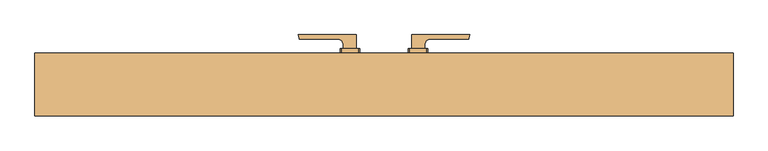
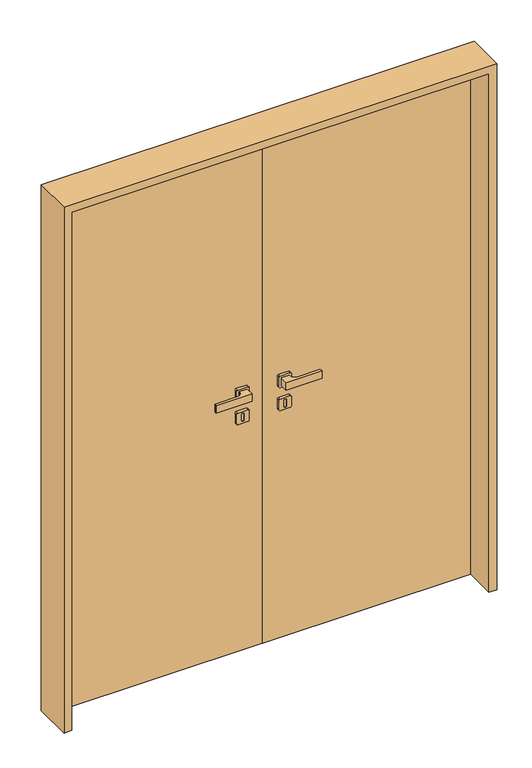
"""IFC4 building model written with IfcOpenShell, lengths in millimetres: door geometry, porta multiplas_growarq : porta giro duplo 80 cm_growarq."""

from ifc_helpers import new_model, si_unit, point, frame, frame_2d, origin, origin_with_axes, place, context, project, spatial, polyline, circle_curve, trimmed, segment, composite_curve, outline, extrude, source, transform, mapped, element, save
from ifc_brep_helpers import plane_surface, cylinder_surface, revolved_surface, advanced_brep


def door_8bf3503e(model_context):
    return source(origin(), model_context, "Body", "SolidModel", [
        advanced_brep(
        [(-61.4752094, 86.0, 975.2140175), (-57.4752094, 86.0, 971.2140175), (-57.4752094, 86.0, 932.3348635), (-61.4752094, 86.0, 928.3348635), (-100.524804, 86.0, 928.3348635), (-104.524804, 86.0, 932.3348635), (-104.524804, 86.0, 971.2071442), (-100.5179308, 86.0, 975.2140175), (-75.9963765, 86.0, 963.1453546), (-86.0064486, 86.0, 963.1453546), (-86.0064486, 86.0, 940.4035264), (-75.9963765, 86.0, 940.4035264), (-61.4752094, 75.0, 975.2140175), (-100.5179308, 75.0, 975.2140175), (-104.524804, 75.0, 971.2071442), (-104.524804, 75.0, 932.3348635), (-100.524804, 75.0, 928.3348635), (-61.4752094, 75.0, 928.3348635), (-57.4752094, 75.0, 932.3348635), (-57.4752094, 75.0, 971.2140175), (-75.9963765, 84.0, 940.4035264), (-86.0064486, 84.0, 940.4035264), (-86.0064486, 84.0, 963.1453546), (-75.9963765, 84.0, 963.1453546)],
        [
            (0, 1, circle_curve(frame((-61.4752094, 86.0, 971.2140175), z_axis=(0.0, 1.0, 0.0), x_axis=(1.0, 0.0, 0.0)), 4.0)),
            (1, 2),
            (2, 3, circle_curve(frame((-61.4752094, 86.0, 932.3348635), z_axis=(0.0, 1.0, 0.0), x_axis=(1.0, 0.0, 0.0)), 4.0)),
            (3, 4),
            (4, 5, circle_curve(frame((-100.524804, 86.0, 932.3348635), z_axis=(0.0, 1.0, 0.0), x_axis=(1.0, 0.0, 0.0)), 4.0)),
            (5, 6),
            (6, 7, circle_curve(frame((-100.5179308, 86.0, 971.2071442), z_axis=(0.0, 1.0, 0.0), x_axis=(1.0, 0.0, 0.0)), 4.0068732)),
            (7, 0),
            (8, 9, circle_curve(frame((-81.0014126, 86.0, 963.1453546), z_axis=(0.0, -1.0, 0.0), x_axis=(1.0, 0.0, 0.0)), 5.0050361)),
            (9, 10),
            (10, 11, circle_curve(frame((-81.0014126, 86.0, 940.4035264), z_axis=(0.0, -1.0, 0.0), x_axis=(1.0, 0.0, 0.0)), 5.0050361)),
            (11, 8),
            (12, 13),
            (13, 14, circle_curve(frame((-100.5179308, 75.0, 971.2071442), z_axis=(0.0, -1.0, 0.0), x_axis=(1.0, 0.0, 0.0)), 4.0068732)),
            (14, 15),
            (15, 16, circle_curve(frame((-100.524804, 75.0, 932.3348635), z_axis=(0.0, -1.0, 0.0), x_axis=(1.0, 0.0, 0.0)), 4.0)),
            (16, 17),
            (17, 18, circle_curve(frame((-61.4752094, 75.0, 932.3348635), z_axis=(0.0, -1.0, 0.0), x_axis=(1.0, 0.0, 0.0)), 4.0)),
            (18, 19),
            (19, 12, circle_curve(frame((-61.4752094, 75.0, 971.2140175), z_axis=(0.0, -1.0, 0.0), x_axis=(1.0, 0.0, 0.0)), 4.0)),
            (7, 13),
            (12, 0),
            (6, 14),
            (5, 15),
            (4, 16),
            (3, 17),
            (2, 18),
            (1, 19),
            (20, 21, circle_curve(frame((-81.0014126, 84.0, 940.4035264), z_axis=(0.0, 1.0, 0.0), x_axis=(1.0, 0.0, 0.0)), 5.0050361)),
            (21, 22),
            (22, 23, circle_curve(frame((-81.0014126, 84.0, 963.1453546), z_axis=(0.0, 1.0, 0.0), x_axis=(1.0, 0.0, 0.0)), 5.0050361)),
            (23, 20),
            (23, 8),
            (11, 20),
            (21, 10),
            (9, 22),
        ],
        [
            plane_surface(frame((-100.5218961, 86.0, 975.2140175), z_axis=(0.0, 1.0, 0.0), x_axis=(-1.0, 0.0, 0.0))),
            plane_surface(frame((-100.5218961, 75.0, 975.2140175), z_axis=(0.0, -1.0, 0.0), x_axis=(1.0, 0.0, 0.0))),
            plane_surface(frame((-61.4752094, 86.0, 975.2140175), z_axis=(0.0, 0.0, 1.0), x_axis=(0.0, -1.0, 0.0))),
            cylinder_surface(frame((-100.5179308, 75.0, 971.2071442), z_axis=(0.0, 1.0, 0.0), x_axis=(1.0, 0.0, 0.0)), 4.0068732),
            plane_surface(frame((-104.524804, 86.0, 971.2071442), z_axis=(-1.0, 0.0, 0.0), x_axis=(0.0, -1.0, 0.0))),
            cylinder_surface(frame((-100.524804, 75.0, 932.3348635), z_axis=(0.0, 1.0, 0.0), x_axis=(1.0, 0.0, 0.0)), 4.0),
            plane_surface(frame((-100.524804, 86.0, 928.3348635), z_axis=(0.0, 0.0, -1.0), x_axis=(0.0, -1.0, 0.0))),
            cylinder_surface(frame((-61.4752094, 75.0, 932.3348635), z_axis=(0.0, 1.0, 0.0), x_axis=(1.0, 0.0, 0.0)), 4.0),
            plane_surface(frame((-57.4752094, 86.0, 932.3348635), z_axis=(1.0, 0.0, 0.0), x_axis=(0.0, -1.0, 0.0))),
            cylinder_surface(frame((-61.4752094, 75.0, 971.2140175), z_axis=(0.0, 1.0, 0.0), x_axis=(1.0, 0.0, 0.0)), 4.0),
            plane_surface(frame((-75.9963765, 84.0, 952.9958878), z_axis=(0.0, 1.0, 0.0), x_axis=(0.0, 0.0, -1.0))),
            plane_surface(frame((-75.9963765, 86.0, 940.4035264), z_axis=(-1.0, 0.0, 0.0), x_axis=(0.0, -1.0, 0.0))),
            plane_surface(frame((-86.0064486, 86.0, 963.1453546), z_axis=(1.0, 0.0, 0.0), x_axis=(0.0, -1.0, 0.0))),
            revolved_surface(polyline([(-75.9963765, 86.0, 940.4035264), (-75.9963765, 84.0, 940.4035264)]), (-81.0014126, 84.0, 940.4035264), (0.0, 1.0, 0.0)),
            revolved_surface(polyline([(-75.9963765, 86.0, 963.1453546), (-75.9963765, 84.0, 963.1453546)]), (-81.0014126, 84.0, 963.1453546), (0.0, 1.0, 0.0)),
        ],
        [
            (0, [[1, 2, 3, 4, 5, 6, 7, 8], [9, 10, 11, 12]]),
            (1, [[13, 14, 15, 16, 17, 18, 19, 20]]),
            (2, [[21, -13, 22, -8]]),
            (3, [[23, -14, -21, -7]]),
            (4, [[24, -15, -23, -6]]),
            (5, [[25, -16, -24, -5]]),
            (6, [[26, -17, -25, -4]]),
            (7, [[27, -18, -26, -3]]),
            (8, [[28, -19, -27, -2]]),
            (9, [[-22, -20, -28, -1]]),
            (10, [[29, 30, 31, 32]]),
            (11, [[33, -12, 34, -32]]),
            (12, [[35, -10, 36, -30]]),
            (13, [[-34, -11, -35, -29]]),
            (14, [[-36, -9, -33, -31]]),
        ],
    ),
        advanced_brep(
        [(-61.4752094, 86.0, 1068.227973), (-57.4752094, 86.0, 1064.227973), (-57.4752094, 86.0, 1025.3488191), (-61.4752094, 86.0, 1021.3488191), (-100.524804, 86.0, 1021.3488191), (-104.524804, 86.0, 1025.3488191), (-104.524804, 86.0, 1064.2210998), (-100.5179308, 86.0, 1068.227973), (-61.4752094, 75.0, 1068.227973), (-100.5179308, 75.0, 1068.227973), (-104.524804, 75.0, 1064.2210998), (-104.524804, 75.0, 1025.3488191), (-100.524804, 75.0, 1021.3488191), (-61.4752094, 75.0, 1021.3488191), (-57.4752094, 75.0, 1025.3488191), (-57.4752094, 75.0, 1064.227973)],
        [
            (0, 1, circle_curve(frame((-61.4752094, 86.0, 1064.227973), z_axis=(0.0, 1.0, 0.0), x_axis=(1.0, 0.0, 0.0)), 4.0)),
            (1, 2),
            (2, 3, circle_curve(frame((-61.4752094, 86.0, 1025.3488191), z_axis=(0.0, 1.0, 0.0), x_axis=(1.0, 0.0, 0.0)), 4.0)),
            (3, 4),
            (4, 5, circle_curve(frame((-100.524804, 86.0, 1025.3488191), z_axis=(0.0, 1.0, 0.0), x_axis=(1.0, 0.0, 0.0)), 4.0)),
            (5, 6),
            (6, 7, circle_curve(frame((-100.5179308, 86.0, 1064.2210998), z_axis=(0.0, 1.0, 0.0), x_axis=(1.0, 0.0, 0.0)), 4.0068732)),
            (7, 0),
            (8, 9),
            (9, 10, circle_curve(frame((-100.5179308, 75.0, 1064.2210998), z_axis=(0.0, -1.0, 0.0), x_axis=(1.0, 0.0, 0.0)), 4.0068732)),
            (10, 11),
            (11, 12, circle_curve(frame((-100.524804, 75.0, 1025.3488191), z_axis=(0.0, -1.0, 0.0), x_axis=(1.0, 0.0, 0.0)), 4.0)),
            (12, 13),
            (13, 14, circle_curve(frame((-61.4752094, 75.0, 1025.3488191), z_axis=(0.0, -1.0, 0.0), x_axis=(1.0, 0.0, 0.0)), 4.0)),
            (14, 15),
            (15, 8, circle_curve(frame((-61.4752094, 75.0, 1064.227973), z_axis=(0.0, -1.0, 0.0), x_axis=(1.0, 0.0, 0.0)), 4.0)),
            (7, 9),
            (8, 0),
            (6, 10),
            (5, 11),
            (4, 12),
            (3, 13),
            (2, 14),
            (1, 15),
        ],
        [
            plane_surface(frame((-100.5218961, 86.0, 975.2140175), z_axis=(0.0, 1.0, 0.0), x_axis=(-1.0, 0.0, 0.0))),
            plane_surface(frame((-100.5218961, 75.0, 975.2140175), z_axis=(0.0, -1.0, 0.0), x_axis=(1.0, 0.0, 0.0))),
            plane_surface(frame((-61.4752094, 86.0, 1068.227973), z_axis=(0.0, 0.0, 1.0), x_axis=(0.0, -1.0, 0.0))),
            cylinder_surface(frame((-100.5179308, 75.0, 1064.2210998), z_axis=(0.0, 1.0, 0.0), x_axis=(1.0, 0.0, 0.0)), 4.0068732),
            plane_surface(frame((-104.524804, 86.0, 1064.2210998), z_axis=(-1.0, 0.0, 0.0), x_axis=(0.0, -1.0, 0.0))),
            cylinder_surface(frame((-100.524804, 75.0, 1025.3488191), z_axis=(0.0, 1.0, 0.0), x_axis=(1.0, 0.0, 0.0)), 4.0),
            plane_surface(frame((-100.524804, 86.0, 1021.3488191), z_axis=(0.0, 0.0, -1.0), x_axis=(0.0, -1.0, 0.0))),
            cylinder_surface(frame((-61.4752094, 75.0, 1025.3488191), z_axis=(0.0, 1.0, 0.0), x_axis=(1.0, 0.0, 0.0)), 4.0),
            plane_surface(frame((-57.4752094, 86.0, 1025.3488191), z_axis=(1.0, 0.0, 0.0), x_axis=(0.0, -1.0, 0.0))),
            cylinder_surface(frame((-61.4752094, 75.0, 1064.227973), z_axis=(0.0, 1.0, 0.0), x_axis=(1.0, 0.0, 0.0)), 4.0),
        ],
        [
            (0, [[1, 2, 3, 4, 5, 6, 7, 8]]),
            (1, [[9, 10, 11, 12, 13, 14, 15, 16]]),
            (2, [[17, -9, 18, -8]]),
            (3, [[19, -10, -17, -7]]),
            (4, [[20, -11, -19, -6]]),
            (5, [[21, -12, -20, -5]]),
            (6, [[22, -13, -21, -4]]),
            (7, [[23, -14, -22, -3]]),
            (8, [[24, -15, -23, -2]]),
            (9, [[-18, -16, -24, -1]]),
        ],
    ),
        extrude(outline(composite_curve([segment(polyline([(-65.4752094, 118.5150355), (-65.4752094, 86.7793682), (-96.524804, 86.7793682), (-96.524804, 93.5981558)]), True, "CONTINUOUS"), segment(trimmed(circle_curve(frame_2d((-111.5516421, 93.5981558)), 15.0268381), [point((-96.524804, 93.5981558))], [point((-111.5516421, 108.6249939))], True, "CARTESIAN"), True, "CONTINUOUS"), segment(polyline([(-111.5516421, 108.6249939), (-200.8409795, 108.6249939)]), True, "CONTINUOUS"), segment(trimmed(circle_curve(frame_2d((-200.8409795, 109.6372538)), 1.0122598), [point((-200.8409795, 108.6249939))], [point((-201.8378608, 109.4614767))], False, "CARTESIAN"), True, "CONTINUOUS"), segment(polyline([(-201.8378608, 109.4614767), (-203.4342475, 118.5150355), (-65.4752094, 118.5150355)]), True, "CONTINUOUS")], self_intersect=False)), frame((0.0, 0.0, 1029.3488191), z_axis=(0.0, 0.0, 1.0), x_axis=(1.0, 0.0, 0.0)), (0.0, 0.0, 1.0), 30.8791539),
        advanced_brep(
        [(-61.4752094, 34.0, 975.2140175), (-100.5179308, 34.0, 975.2140175), (-104.524804, 34.0, 971.2071442), (-104.524804, 34.0, 932.3348635), (-100.524804, 34.0, 928.3348635), (-61.4752094, 34.0, 928.3348635), (-57.4752094, 34.0, 932.3348635), (-57.4752094, 34.0, 971.2140175), (-75.9963765, 34.0, 963.1453546), (-75.9963765, 34.0, 940.4035264), (-86.0064486, 34.0, 940.4035264), (-86.0064486, 34.0, 963.1453546), (-61.4752094, 45.0, 975.2140175), (-57.4752094, 45.0, 971.2140175), (-57.4752094, 45.0, 932.3348635), (-61.4752094, 45.0, 928.3348635), (-100.524804, 45.0, 928.3348635), (-104.524804, 45.0, 932.3348635), (-104.524804, 45.0, 971.2071442), (-100.5179308, 45.0, 975.2140175), (-75.9963765, 36.0, 940.4035264), (-75.9963765, 36.0, 963.1453546), (-86.0064486, 36.0, 963.1453546), (-86.0064486, 36.0, 940.4035264)],
        [
            (0, 1),
            (1, 2, circle_curve(frame((-100.5179308, 34.0, 971.2071442), z_axis=(0.0, -1.0, 0.0), x_axis=(1.0, 0.0, 0.0)), 4.0068732)),
            (2, 3),
            (3, 4, circle_curve(frame((-100.524804, 34.0, 932.3348635), z_axis=(0.0, -1.0, 0.0), x_axis=(1.0, 0.0, 0.0)), 4.0)),
            (4, 5),
            (5, 6, circle_curve(frame((-61.4752094, 34.0, 932.3348635), z_axis=(0.0, -1.0, 0.0), x_axis=(1.0, 0.0, 0.0)), 4.0)),
            (6, 7),
            (7, 0, circle_curve(frame((-61.4752094, 34.0, 971.2140175), z_axis=(0.0, -1.0, 0.0), x_axis=(1.0, 0.0, 0.0)), 4.0)),
            (8, 9),
            (9, 10, circle_curve(frame((-81.0014126, 34.0, 940.4035264), z_axis=(0.0, 1.0, 0.0), x_axis=(1.0, 0.0, 0.0)), 5.0050361)),
            (10, 11),
            (11, 8, circle_curve(frame((-81.0014126, 34.0, 963.1453546), z_axis=(0.0, 1.0, 0.0), x_axis=(1.0, 0.0, 0.0)), 5.0050361)),
            (12, 13, circle_curve(frame((-61.4752094, 45.0, 971.2140175), z_axis=(0.0, 1.0, 0.0), x_axis=(1.0, 0.0, 0.0)), 4.0)),
            (13, 14),
            (14, 15, circle_curve(frame((-61.4752094, 45.0, 932.3348635), z_axis=(0.0, 1.0, 0.0), x_axis=(1.0, 0.0, 0.0)), 4.0)),
            (15, 16),
            (16, 17, circle_curve(frame((-100.524804, 45.0, 932.3348635), z_axis=(0.0, 1.0, 0.0), x_axis=(1.0, 0.0, 0.0)), 4.0)),
            (17, 18),
            (18, 19, circle_curve(frame((-100.5179308, 45.0, 971.2071442), z_axis=(0.0, 1.0, 0.0), x_axis=(1.0, 0.0, 0.0)), 4.0068732)),
            (19, 12),
            (0, 12),
            (19, 1),
            (18, 2),
            (17, 3),
            (16, 4),
            (15, 5),
            (14, 6),
            (13, 7),
            (20, 21),
            (21, 22, circle_curve(frame((-81.0014126, 36.0, 963.1453546), z_axis=(0.0, -1.0, 0.0), x_axis=(1.0, 0.0, 0.0)), 5.0050361)),
            (22, 23),
            (23, 20, circle_curve(frame((-81.0014126, 36.0, 940.4035264), z_axis=(0.0, -1.0, 0.0), x_axis=(1.0, 0.0, 0.0)), 5.0050361)),
            (20, 9),
            (8, 21),
            (22, 11),
            (10, 23),
        ],
        [
            plane_surface(frame((-100.5218961, 34.0, 975.2140175), z_axis=(0.0, -1.0, 0.0), x_axis=(-1.0, 0.0, 0.0))),
            plane_surface(frame((-100.5218961, 45.0, 975.2140175), z_axis=(0.0, 1.0, 0.0), x_axis=(1.0, 0.0, 0.0))),
            plane_surface(frame((-61.4752094, 34.0, 975.2140175), z_axis=(0.0, 0.0, 1.0), x_axis=(0.0, 1.0, 0.0))),
            cylinder_surface(frame((-100.5179308, 45.0, 971.2071442), z_axis=(0.0, -1.0, 0.0), x_axis=(1.0, 0.0, 0.0)), 4.0068732),
            plane_surface(frame((-104.524804, 34.0, 971.2071442), z_axis=(-1.0, 0.0, 0.0), x_axis=(0.0, 1.0, 0.0))),
            cylinder_surface(frame((-100.524804, 45.0, 932.3348635), z_axis=(0.0, -1.0, 0.0), x_axis=(1.0, 0.0, 0.0)), 4.0),
            plane_surface(frame((-100.524804, 34.0, 928.3348635), z_axis=(0.0, 0.0, -1.0), x_axis=(0.0, 1.0, 0.0))),
            cylinder_surface(frame((-61.4752094, 45.0, 932.3348635), z_axis=(0.0, -1.0, 0.0), x_axis=(1.0, 0.0, 0.0)), 4.0),
            plane_surface(frame((-57.4752094, 34.0, 932.3348635), z_axis=(1.0, 0.0, 0.0), x_axis=(0.0, 1.0, 0.0))),
            cylinder_surface(frame((-61.4752094, 45.0, 971.2140175), z_axis=(0.0, -1.0, 0.0), x_axis=(1.0, 0.0, 0.0)), 4.0),
            plane_surface(frame((-75.9963765, 36.0, 952.9958878), z_axis=(0.0, -1.0, 0.0), x_axis=(0.0, 0.0, -1.0))),
            plane_surface(frame((-75.9963765, 34.0, 940.4035264), z_axis=(-1.0, 0.0, 0.0), x_axis=(0.0, 1.0, 0.0))),
            plane_surface(frame((-86.0064486, 34.0, 963.1453546), z_axis=(1.0, 0.0, 0.0), x_axis=(0.0, 1.0, 0.0))),
            revolved_surface(polyline([(-75.9963765, 34.0, 940.4035264), (-75.9963765, 36.0, 940.4035264)]), (-81.0014126, 36.0, 940.4035264), (0.0, -1.0, 0.0)),
            revolved_surface(polyline([(-75.9963765, 34.0, 963.1453546), (-75.9963765, 36.0, 963.1453546)]), (-81.0014126, 36.0, 963.1453546), (0.0, -1.0, 0.0)),
        ],
        [
            (0, [[1, 2, 3, 4, 5, 6, 7, 8], [9, 10, 11, 12]]),
            (1, [[13, 14, 15, 16, 17, 18, 19, 20]]),
            (2, [[-1, 21, -20, 22]]),
            (3, [[-2, -22, -19, 23]]),
            (4, [[-3, -23, -18, 24]]),
            (5, [[-4, -24, -17, 25]]),
            (6, [[-5, -25, -16, 26]]),
            (7, [[-6, -26, -15, 27]]),
            (8, [[-7, -27, -14, 28]]),
            (9, [[-8, -28, -13, -21]]),
            (10, [[29, 30, 31, 32]]),
            (11, [[-29, 33, -9, 34]]),
            (12, [[-31, 35, -11, 36]]),
            (13, [[-32, -36, -10, -33]]),
            (14, [[-30, -34, -12, -35]]),
        ],
    ),
        advanced_brep(
        [(-61.4752094, 34.0, 1068.227973), (-100.5179308, 34.0, 1068.227973), (-104.524804, 34.0, 1064.2210998), (-104.524804, 34.0, 1025.3488191), (-100.524804, 34.0, 1021.3488191), (-61.4752094, 34.0, 1021.3488191), (-57.4752094, 34.0, 1025.3488191), (-57.4752094, 34.0, 1064.227973), (-61.4752094, 45.0, 1068.227973), (-57.4752094, 45.0, 1064.227973), (-57.4752094, 45.0, 1025.3488191), (-61.4752094, 45.0, 1021.3488191), (-100.524804, 45.0, 1021.3488191), (-104.524804, 45.0, 1025.3488191), (-104.524804, 45.0, 1064.2210998), (-100.5179308, 45.0, 1068.227973)],
        [
            (0, 1),
            (1, 2, circle_curve(frame((-100.5179308, 34.0, 1064.2210998), z_axis=(0.0, -1.0, 0.0), x_axis=(1.0, 0.0, 0.0)), 4.0068732)),
            (2, 3),
            (3, 4, circle_curve(frame((-100.524804, 34.0, 1025.3488191), z_axis=(0.0, -1.0, 0.0), x_axis=(1.0, 0.0, 0.0)), 4.0)),
            (4, 5),
            (5, 6, circle_curve(frame((-61.4752094, 34.0, 1025.3488191), z_axis=(0.0, -1.0, 0.0), x_axis=(1.0, 0.0, 0.0)), 4.0)),
            (6, 7),
            (7, 0, circle_curve(frame((-61.4752094, 34.0, 1064.227973), z_axis=(0.0, -1.0, 0.0), x_axis=(1.0, 0.0, 0.0)), 4.0)),
            (8, 9, circle_curve(frame((-61.4752094, 45.0, 1064.227973), z_axis=(0.0, 1.0, 0.0), x_axis=(1.0, 0.0, 0.0)), 4.0)),
            (9, 10),
            (10, 11, circle_curve(frame((-61.4752094, 45.0, 1025.3488191), z_axis=(0.0, 1.0, 0.0), x_axis=(1.0, 0.0, 0.0)), 4.0)),
            (11, 12),
            (12, 13, circle_curve(frame((-100.524804, 45.0, 1025.3488191), z_axis=(0.0, 1.0, 0.0), x_axis=(1.0, 0.0, 0.0)), 4.0)),
            (13, 14),
            (14, 15, circle_curve(frame((-100.5179308, 45.0, 1064.2210998), z_axis=(0.0, 1.0, 0.0), x_axis=(1.0, 0.0, 0.0)), 4.0068732)),
            (15, 8),
            (0, 8),
            (15, 1),
            (14, 2),
            (13, 3),
            (12, 4),
            (11, 5),
            (10, 6),
            (9, 7),
        ],
        [
            plane_surface(frame((-100.5218961, 34.0, 975.2140175), z_axis=(0.0, -1.0, 0.0), x_axis=(-1.0, 0.0, 0.0))),
            plane_surface(frame((-100.5218961, 45.0, 975.2140175), z_axis=(0.0, 1.0, 0.0), x_axis=(1.0, 0.0, 0.0))),
            plane_surface(frame((-61.4752094, 34.0, 1068.227973), z_axis=(0.0, 0.0, 1.0), x_axis=(0.0, 1.0, 0.0))),
            cylinder_surface(frame((-100.5179308, 45.0, 1064.2210998), z_axis=(0.0, -1.0, 0.0), x_axis=(1.0, 0.0, 0.0)), 4.0068732),
            plane_surface(frame((-104.524804, 34.0, 1064.2210998), z_axis=(-1.0, 0.0, 0.0), x_axis=(0.0, 1.0, 0.0))),
            cylinder_surface(frame((-100.524804, 45.0, 1025.3488191), z_axis=(0.0, -1.0, 0.0), x_axis=(1.0, 0.0, 0.0)), 4.0),
            plane_surface(frame((-100.524804, 34.0, 1021.3488191), z_axis=(0.0, 0.0, -1.0), x_axis=(0.0, 1.0, 0.0))),
            cylinder_surface(frame((-61.4752094, 45.0, 1025.3488191), z_axis=(0.0, -1.0, 0.0), x_axis=(1.0, 0.0, 0.0)), 4.0),
            plane_surface(frame((-57.4752094, 34.0, 1025.3488191), z_axis=(1.0, 0.0, 0.0), x_axis=(0.0, 1.0, 0.0))),
            cylinder_surface(frame((-61.4752094, 45.0, 1064.227973), z_axis=(0.0, -1.0, 0.0), x_axis=(1.0, 0.0, 0.0)), 4.0),
        ],
        [
            (0, [[1, 2, 3, 4, 5, 6, 7, 8]]),
            (1, [[9, 10, 11, 12, 13, 14, 15, 16]]),
            (2, [[-1, 17, -16, 18]]),
            (3, [[-2, -18, -15, 19]]),
            (4, [[-3, -19, -14, 20]]),
            (5, [[-4, -20, -13, 21]]),
            (6, [[-5, -21, -12, 22]]),
            (7, [[-6, -22, -11, 23]]),
            (8, [[-7, -23, -10, 24]]),
            (9, [[-8, -24, -9, -17]]),
        ],
    ),
        extrude(outline(composite_curve([segment(polyline([(-65.4752094, 1.4849645), (-203.4342475, 1.4849645), (-201.8378608, 10.5385233)]), True, "CONTINUOUS"), segment(trimmed(circle_curve(frame_2d((-200.8409795, 10.3627462)), 1.0122598), [point((-201.8378608, 10.5385233))], [point((-200.8409795, 11.3750061))], False, "CARTESIAN"), True, "CONTINUOUS"), segment(polyline([(-200.8409795, 11.3750061), (-111.5516421, 11.3750061)]), True, "CONTINUOUS"), segment(trimmed(circle_curve(frame_2d((-111.5516421, 26.4018442)), 15.0268381), [point((-111.5516421, 11.3750061))], [point((-96.524804, 26.4018442))], True, "CARTESIAN"), True, "CONTINUOUS"), segment(polyline([(-96.524804, 26.4018442), (-96.524804, 33.2206318), (-65.4752094, 33.2206318), (-65.4752094, 1.4849645)]), True, "CONTINUOUS")], self_intersect=False)), frame((0.0, 0.0, 1029.3488191), z_axis=(0.0, 0.0, 1.0), x_axis=(1.0, 0.0, 0.0)), (0.0, 0.0, 1.0), 30.8791539),
        extrude(outline(polyline([(-1.0, 45.0), (-798.0, 45.0), (-798.0, 75.0), (-1.0, 75.0), (-1.0, 45.0)])), origin_with_axes(), (0.0, 0.0, 1.0), 2098.0),
        advanced_brep(
        [(61.4752094, 86.0, 975.2140175), (100.5179308, 86.0, 975.2140175), (104.524804, 86.0, 971.2071442), (104.524804, 86.0, 932.3348635), (100.524804, 86.0, 928.3348635), (61.4752094, 86.0, 928.3348635), (57.4752094, 86.0, 932.3348635), (57.4752094, 86.0, 971.2140175), (75.9963765, 86.0, 963.1453546), (75.9963765, 86.0, 940.4035264), (86.0064486, 86.0, 940.4035264), (86.0064486, 86.0, 963.1453546), (61.4752094, 75.0, 975.2140175), (57.4752094, 75.0, 971.2140175), (57.4752094, 75.0, 932.3348635), (61.4752094, 75.0, 928.3348635), (100.524804, 75.0, 928.3348635), (104.524804, 75.0, 932.3348635), (104.524804, 75.0, 971.2071442), (100.5179308, 75.0, 975.2140175), (75.9963765, 84.0, 940.4035264), (75.9963765, 84.0, 963.1453546), (86.0064486, 84.0, 963.1453546), (86.0064486, 84.0, 940.4035264)],
        [
            (0, 1),
            (1, 2, circle_curve(frame((100.5179308, 86.0, 971.2071442), z_axis=(0.0, 1.0, 0.0), x_axis=(-1.0, 0.0, 0.0)), 4.0068732)),
            (2, 3),
            (3, 4, circle_curve(frame((100.524804, 86.0, 932.3348635), z_axis=(0.0, 1.0, 0.0), x_axis=(-1.0, 0.0, 0.0)), 4.0)),
            (4, 5),
            (5, 6, circle_curve(frame((61.4752094, 86.0, 932.3348635), z_axis=(0.0, 1.0, 0.0), x_axis=(-1.0, 0.0, 0.0)), 4.0)),
            (6, 7),
            (7, 0, circle_curve(frame((61.4752094, 86.0, 971.2140175), z_axis=(0.0, 1.0, 0.0), x_axis=(-1.0, 0.0, 0.0)), 4.0)),
            (8, 9),
            (9, 10, circle_curve(frame((81.0014126, 86.0, 940.4035264), z_axis=(0.0, -1.0, 0.0), x_axis=(-1.0, 0.0, 0.0)), 5.0050361)),
            (10, 11),
            (11, 8, circle_curve(frame((81.0014126, 86.0, 963.1453546), z_axis=(0.0, -1.0, 0.0), x_axis=(-1.0, 0.0, 0.0)), 5.0050361)),
            (12, 13, circle_curve(frame((61.4752094, 75.0, 971.2140175), z_axis=(0.0, -1.0, 0.0), x_axis=(-1.0, 0.0, 0.0)), 4.0)),
            (13, 14),
            (14, 15, circle_curve(frame((61.4752094, 75.0, 932.3348635), z_axis=(0.0, -1.0, 0.0), x_axis=(-1.0, 0.0, 0.0)), 4.0)),
            (15, 16),
            (16, 17, circle_curve(frame((100.524804, 75.0, 932.3348635), z_axis=(0.0, -1.0, 0.0), x_axis=(-1.0, 0.0, 0.0)), 4.0)),
            (17, 18),
            (18, 19, circle_curve(frame((100.5179308, 75.0, 971.2071442), z_axis=(0.0, -1.0, 0.0), x_axis=(-1.0, 0.0, 0.0)), 4.0068732)),
            (19, 12),
            (0, 12),
            (19, 1),
            (18, 2),
            (17, 3),
            (16, 4),
            (15, 5),
            (14, 6),
            (13, 7),
            (20, 21),
            (21, 22, circle_curve(frame((81.0014126, 84.0, 963.1453546), z_axis=(0.0, 1.0, 0.0), x_axis=(-1.0, 0.0, 0.0)), 5.0050361)),
            (22, 23),
            (23, 20, circle_curve(frame((81.0014126, 84.0, 940.4035264), z_axis=(0.0, 1.0, 0.0), x_axis=(-1.0, 0.0, 0.0)), 5.0050361)),
            (20, 9),
            (8, 21),
            (22, 11),
            (10, 23),
        ],
        [
            plane_surface(frame((100.5218961, 86.0, 975.2140175), z_axis=(0.0, 1.0, 0.0), x_axis=(1.0, 0.0, 0.0))),
            plane_surface(frame((100.5218961, 75.0, 975.2140175), z_axis=(0.0, -1.0, 0.0), x_axis=(-1.0, 0.0, 0.0))),
            plane_surface(frame((61.4752094, 86.0, 975.2140175), z_axis=(0.0, 0.0, 1.0), x_axis=(0.0, -1.0, 0.0))),
            cylinder_surface(frame((100.5179308, 75.0, 971.2071442), z_axis=(0.0, 1.0, 0.0), x_axis=(-1.0, 0.0, 0.0)), 4.0068732),
            plane_surface(frame((104.524804, 86.0, 971.2071442), z_axis=(1.0, 0.0, 0.0), x_axis=(0.0, -1.0, 0.0))),
            cylinder_surface(frame((100.524804, 75.0, 932.3348635), z_axis=(0.0, 1.0, 0.0), x_axis=(-1.0, 0.0, 0.0)), 4.0),
            plane_surface(frame((100.524804, 86.0, 928.3348635), z_axis=(0.0, 0.0, -1.0), x_axis=(0.0, -1.0, 0.0))),
            cylinder_surface(frame((61.4752094, 75.0, 932.3348635), z_axis=(0.0, 1.0, 0.0), x_axis=(-1.0, 0.0, 0.0)), 4.0),
            plane_surface(frame((57.4752094, 86.0, 932.3348635), z_axis=(-1.0, 0.0, 0.0), x_axis=(0.0, -1.0, 0.0))),
            cylinder_surface(frame((61.4752094, 75.0, 971.2140175), z_axis=(0.0, 1.0, 0.0), x_axis=(-1.0, 0.0, 0.0)), 4.0),
            plane_surface(frame((75.9963765, 84.0, 952.9958878), z_axis=(0.0, 1.0, 0.0), x_axis=(0.0, 0.0, -1.0))),
            plane_surface(frame((75.9963765, 86.0, 940.4035264), z_axis=(1.0, 0.0, 0.0), x_axis=(0.0, -1.0, 0.0))),
            plane_surface(frame((86.0064486, 86.0, 963.1453546), z_axis=(-1.0, 0.0, 0.0), x_axis=(0.0, -1.0, 0.0))),
            revolved_surface(polyline([(75.9963765, 86.0, 940.4035264), (75.9963765, 84.0, 940.4035264)]), (81.0014126, 84.0, 940.4035264), (0.0, 1.0, 0.0)),
            revolved_surface(polyline([(75.9963765, 86.0, 963.1453546), (75.9963765, 84.0, 963.1453546)]), (81.0014126, 84.0, 963.1453546), (0.0, 1.0, 0.0)),
        ],
        [
            (0, [[1, 2, 3, 4, 5, 6, 7, 8], [9, 10, 11, 12]]),
            (1, [[13, 14, 15, 16, 17, 18, 19, 20]]),
            (2, [[-1, 21, -20, 22]]),
            (3, [[-2, -22, -19, 23]]),
            (4, [[-3, -23, -18, 24]]),
            (5, [[-4, -24, -17, 25]]),
            (6, [[-5, -25, -16, 26]]),
            (7, [[-6, -26, -15, 27]]),
            (8, [[-7, -27, -14, 28]]),
            (9, [[-8, -28, -13, -21]]),
            (10, [[29, 30, 31, 32]]),
            (11, [[-29, 33, -9, 34]]),
            (12, [[-31, 35, -11, 36]]),
            (13, [[-32, -36, -10, -33]]),
            (14, [[-30, -34, -12, -35]]),
        ],
    ),
        advanced_brep(
        [(61.4752094, 86.0, 1068.227973), (100.5179308, 86.0, 1068.227973), (104.524804, 86.0, 1064.2210998), (104.524804, 86.0, 1025.3488191), (100.524804, 86.0, 1021.3488191), (61.4752094, 86.0, 1021.3488191), (57.4752094, 86.0, 1025.3488191), (57.4752094, 86.0, 1064.227973), (61.4752094, 75.0, 1068.227973), (57.4752094, 75.0, 1064.227973), (57.4752094, 75.0, 1025.3488191), (61.4752094, 75.0, 1021.3488191), (100.524804, 75.0, 1021.3488191), (104.524804, 75.0, 1025.3488191), (104.524804, 75.0, 1064.2210998), (100.5179308, 75.0, 1068.227973)],
        [
            (0, 1),
            (1, 2, circle_curve(frame((100.5179308, 86.0, 1064.2210998), z_axis=(0.0, 1.0, 0.0), x_axis=(-1.0, 0.0, 0.0)), 4.0068732)),
            (2, 3),
            (3, 4, circle_curve(frame((100.524804, 86.0, 1025.3488191), z_axis=(0.0, 1.0, 0.0), x_axis=(-1.0, 0.0, 0.0)), 4.0)),
            (4, 5),
            (5, 6, circle_curve(frame((61.4752094, 86.0, 1025.3488191), z_axis=(0.0, 1.0, 0.0), x_axis=(-1.0, 0.0, 0.0)), 4.0)),
            (6, 7),
            (7, 0, circle_curve(frame((61.4752094, 86.0, 1064.227973), z_axis=(0.0, 1.0, 0.0), x_axis=(-1.0, 0.0, 0.0)), 4.0)),
            (8, 9, circle_curve(frame((61.4752094, 75.0, 1064.227973), z_axis=(0.0, -1.0, 0.0), x_axis=(-1.0, 0.0, 0.0)), 4.0)),
            (9, 10),
            (10, 11, circle_curve(frame((61.4752094, 75.0, 1025.3488191), z_axis=(0.0, -1.0, 0.0), x_axis=(-1.0, 0.0, 0.0)), 4.0)),
            (11, 12),
            (12, 13, circle_curve(frame((100.524804, 75.0, 1025.3488191), z_axis=(0.0, -1.0, 0.0), x_axis=(-1.0, 0.0, 0.0)), 4.0)),
            (13, 14),
            (14, 15, circle_curve(frame((100.5179308, 75.0, 1064.2210998), z_axis=(0.0, -1.0, 0.0), x_axis=(-1.0, 0.0, 0.0)), 4.0068732)),
            (15, 8),
            (0, 8),
            (15, 1),
            (14, 2),
            (13, 3),
            (12, 4),
            (11, 5),
            (10, 6),
            (9, 7),
        ],
        [
            plane_surface(frame((100.5218961, 86.0, 975.2140175), z_axis=(0.0, 1.0, 0.0), x_axis=(1.0, 0.0, 0.0))),
            plane_surface(frame((100.5218961, 75.0, 975.2140175), z_axis=(0.0, -1.0, 0.0), x_axis=(-1.0, 0.0, 0.0))),
            plane_surface(frame((61.4752094, 86.0, 1068.227973), z_axis=(0.0, 0.0, 1.0), x_axis=(0.0, -1.0, 0.0))),
            cylinder_surface(frame((100.5179308, 75.0, 1064.2210998), z_axis=(0.0, 1.0, 0.0), x_axis=(-1.0, 0.0, 0.0)), 4.0068732),
            plane_surface(frame((104.524804, 86.0, 1064.2210998), z_axis=(1.0, 0.0, 0.0), x_axis=(0.0, -1.0, 0.0))),
            cylinder_surface(frame((100.524804, 75.0, 1025.3488191), z_axis=(0.0, 1.0, 0.0), x_axis=(-1.0, 0.0, 0.0)), 4.0),
            plane_surface(frame((100.524804, 86.0, 1021.3488191), z_axis=(0.0, 0.0, -1.0), x_axis=(0.0, -1.0, 0.0))),
            cylinder_surface(frame((61.4752094, 75.0, 1025.3488191), z_axis=(0.0, 1.0, 0.0), x_axis=(-1.0, 0.0, 0.0)), 4.0),
            plane_surface(frame((57.4752094, 86.0, 1025.3488191), z_axis=(-1.0, 0.0, 0.0), x_axis=(0.0, -1.0, 0.0))),
            cylinder_surface(frame((61.4752094, 75.0, 1064.227973), z_axis=(0.0, 1.0, 0.0), x_axis=(-1.0, 0.0, 0.0)), 4.0),
        ],
        [
            (0, [[1, 2, 3, 4, 5, 6, 7, 8]]),
            (1, [[9, 10, 11, 12, 13, 14, 15, 16]]),
            (2, [[-1, 17, -16, 18]]),
            (3, [[-2, -18, -15, 19]]),
            (4, [[-3, -19, -14, 20]]),
            (5, [[-4, -20, -13, 21]]),
            (6, [[-5, -21, -12, 22]]),
            (7, [[-6, -22, -11, 23]]),
            (8, [[-7, -23, -10, 24]]),
            (9, [[-8, -24, -9, -17]]),
        ],
    ),
        extrude(outline(composite_curve([segment(polyline([(65.4752094, 118.5150355), (203.4342475, 118.5150355), (201.8378608, 109.4614767)]), True, "CONTINUOUS"), segment(trimmed(circle_curve(frame_2d((200.8409795, 109.6372538)), 1.0122598), [point((201.8378608, 109.4614767))], [point((200.8409795, 108.6249939))], False, "CARTESIAN"), True, "CONTINUOUS"), segment(polyline([(200.8409795, 108.6249939), (111.5516421, 108.6249939)]), True, "CONTINUOUS"), segment(trimmed(circle_curve(frame_2d((111.5516421, 93.5981558)), 15.0268381), [point((111.5516421, 108.6249939))], [point((96.524804, 93.5981558))], True, "CARTESIAN"), True, "CONTINUOUS"), segment(polyline([(96.524804, 93.5981558), (96.524804, 86.7793682), (65.4752094, 86.7793682), (65.4752094, 118.5150355)]), True, "CONTINUOUS")], self_intersect=False)), frame((0.0, 0.0, 1029.3488191), z_axis=(0.0, 0.0, 1.0), x_axis=(1.0, 0.0, 0.0)), (0.0, 0.0, 1.0), 30.8791539),
        advanced_brep(
        [(61.4752094, 34.0, 975.2140175), (57.4752094, 34.0, 971.2140175), (57.4752094, 34.0, 932.3348635), (61.4752094, 34.0, 928.3348635), (100.524804, 34.0, 928.3348635), (104.524804, 34.0, 932.3348635), (104.524804, 34.0, 971.2071442), (100.5179308, 34.0, 975.2140175), (75.9963765, 34.0, 963.1453546), (86.0064486, 34.0, 963.1453546), (86.0064486, 34.0, 940.4035264), (75.9963765, 34.0, 940.4035264), (61.4752094, 45.0, 975.2140175), (100.5179308, 45.0, 975.2140175), (104.524804, 45.0, 971.2071442), (104.524804, 45.0, 932.3348635), (100.524804, 45.0, 928.3348635), (61.4752094, 45.0, 928.3348635), (57.4752094, 45.0, 932.3348635), (57.4752094, 45.0, 971.2140175), (75.9963765, 36.0, 940.4035264), (86.0064486, 36.0, 940.4035264), (86.0064486, 36.0, 963.1453546), (75.9963765, 36.0, 963.1453546)],
        [
            (0, 1, circle_curve(frame((61.4752094, 34.0, 971.2140175), z_axis=(0.0, -1.0, 0.0), x_axis=(-1.0, 0.0, 0.0)), 4.0)),
            (1, 2),
            (2, 3, circle_curve(frame((61.4752094, 34.0, 932.3348635), z_axis=(0.0, -1.0, 0.0), x_axis=(-1.0, 0.0, 0.0)), 4.0)),
            (3, 4),
            (4, 5, circle_curve(frame((100.524804, 34.0, 932.3348635), z_axis=(0.0, -1.0, 0.0), x_axis=(-1.0, 0.0, 0.0)), 4.0)),
            (5, 6),
            (6, 7, circle_curve(frame((100.5179308, 34.0, 971.2071442), z_axis=(0.0, -1.0, 0.0), x_axis=(-1.0, 0.0, 0.0)), 4.0068732)),
            (7, 0),
            (8, 9, circle_curve(frame((81.0014126, 34.0, 963.1453546), z_axis=(0.0, 1.0, 0.0), x_axis=(-1.0, 0.0, 0.0)), 5.0050361)),
            (9, 10),
            (10, 11, circle_curve(frame((81.0014126, 34.0, 940.4035264), z_axis=(0.0, 1.0, 0.0), x_axis=(-1.0, 0.0, 0.0)), 5.0050361)),
            (11, 8),
            (12, 13),
            (13, 14, circle_curve(frame((100.5179308, 45.0, 971.2071442), z_axis=(0.0, 1.0, 0.0), x_axis=(-1.0, 0.0, 0.0)), 4.0068732)),
            (14, 15),
            (15, 16, circle_curve(frame((100.524804, 45.0, 932.3348635), z_axis=(0.0, 1.0, 0.0), x_axis=(-1.0, 0.0, 0.0)), 4.0)),
            (16, 17),
            (17, 18, circle_curve(frame((61.4752094, 45.0, 932.3348635), z_axis=(0.0, 1.0, 0.0), x_axis=(-1.0, 0.0, 0.0)), 4.0)),
            (18, 19),
            (19, 12, circle_curve(frame((61.4752094, 45.0, 971.2140175), z_axis=(0.0, 1.0, 0.0), x_axis=(-1.0, 0.0, 0.0)), 4.0)),
            (7, 13),
            (12, 0),
            (6, 14),
            (5, 15),
            (4, 16),
            (3, 17),
            (2, 18),
            (1, 19),
            (20, 21, circle_curve(frame((81.0014126, 36.0, 940.4035264), z_axis=(0.0, -1.0, 0.0), x_axis=(-1.0, 0.0, 0.0)), 5.0050361)),
            (21, 22),
            (22, 23, circle_curve(frame((81.0014126, 36.0, 963.1453546), z_axis=(0.0, -1.0, 0.0), x_axis=(-1.0, 0.0, 0.0)), 5.0050361)),
            (23, 20),
            (23, 8),
            (11, 20),
            (21, 10),
            (9, 22),
        ],
        [
            plane_surface(frame((100.5218961, 34.0, 975.2140175), z_axis=(0.0, -1.0, 0.0), x_axis=(1.0, 0.0, 0.0))),
            plane_surface(frame((100.5218961, 45.0, 975.2140175), z_axis=(0.0, 1.0, 0.0), x_axis=(-1.0, 0.0, 0.0))),
            plane_surface(frame((61.4752094, 34.0, 975.2140175), z_axis=(0.0, 0.0, 1.0), x_axis=(0.0, 1.0, 0.0))),
            cylinder_surface(frame((100.5179308, 45.0, 971.2071442), z_axis=(0.0, -1.0, 0.0), x_axis=(-1.0, 0.0, 0.0)), 4.0068732),
            plane_surface(frame((104.524804, 34.0, 971.2071442), z_axis=(1.0, 0.0, 0.0), x_axis=(0.0, 1.0, 0.0))),
            cylinder_surface(frame((100.524804, 45.0, 932.3348635), z_axis=(0.0, -1.0, 0.0), x_axis=(-1.0, 0.0, 0.0)), 4.0),
            plane_surface(frame((100.524804, 34.0, 928.3348635), z_axis=(0.0, 0.0, -1.0), x_axis=(0.0, 1.0, 0.0))),
            cylinder_surface(frame((61.4752094, 45.0, 932.3348635), z_axis=(0.0, -1.0, 0.0), x_axis=(-1.0, 0.0, 0.0)), 4.0),
            plane_surface(frame((57.4752094, 34.0, 932.3348635), z_axis=(-1.0, 0.0, 0.0), x_axis=(0.0, 1.0, 0.0))),
            cylinder_surface(frame((61.4752094, 45.0, 971.2140175), z_axis=(0.0, -1.0, 0.0), x_axis=(-1.0, 0.0, 0.0)), 4.0),
            plane_surface(frame((75.9963765, 36.0, 952.9958878), z_axis=(0.0, -1.0, 0.0), x_axis=(0.0, 0.0, -1.0))),
            plane_surface(frame((75.9963765, 34.0, 940.4035264), z_axis=(1.0, 0.0, 0.0), x_axis=(0.0, 1.0, 0.0))),
            plane_surface(frame((86.0064486, 34.0, 963.1453546), z_axis=(-1.0, 0.0, 0.0), x_axis=(0.0, 1.0, 0.0))),
            revolved_surface(polyline([(75.9963765, 34.0, 940.4035264), (75.9963765, 36.0, 940.4035264)]), (81.0014126, 36.0, 940.4035264), (0.0, -1.0, 0.0)),
            revolved_surface(polyline([(75.9963765, 34.0, 963.1453546), (75.9963765, 36.0, 963.1453546)]), (81.0014126, 36.0, 963.1453546), (0.0, -1.0, 0.0)),
        ],
        [
            (0, [[1, 2, 3, 4, 5, 6, 7, 8], [9, 10, 11, 12]]),
            (1, [[13, 14, 15, 16, 17, 18, 19, 20]]),
            (2, [[21, -13, 22, -8]]),
            (3, [[23, -14, -21, -7]]),
            (4, [[24, -15, -23, -6]]),
            (5, [[25, -16, -24, -5]]),
            (6, [[26, -17, -25, -4]]),
            (7, [[27, -18, -26, -3]]),
            (8, [[28, -19, -27, -2]]),
            (9, [[-22, -20, -28, -1]]),
            (10, [[29, 30, 31, 32]]),
            (11, [[33, -12, 34, -32]]),
            (12, [[35, -10, 36, -30]]),
            (13, [[-34, -11, -35, -29]]),
            (14, [[-36, -9, -33, -31]]),
        ],
    ),
        advanced_brep(
        [(61.4752094, 34.0, 1068.227973), (57.4752094, 34.0, 1064.227973), (57.4752094, 34.0, 1025.3488191), (61.4752094, 34.0, 1021.3488191), (100.524804, 34.0, 1021.3488191), (104.524804, 34.0, 1025.3488191), (104.524804, 34.0, 1064.2210998), (100.5179308, 34.0, 1068.227973), (61.4752094, 45.0, 1068.227973), (100.5179308, 45.0, 1068.227973), (104.524804, 45.0, 1064.2210998), (104.524804, 45.0, 1025.3488191), (100.524804, 45.0, 1021.3488191), (61.4752094, 45.0, 1021.3488191), (57.4752094, 45.0, 1025.3488191), (57.4752094, 45.0, 1064.227973)],
        [
            (0, 1, circle_curve(frame((61.4752094, 34.0, 1064.227973), z_axis=(0.0, -1.0, 0.0), x_axis=(-1.0, 0.0, 0.0)), 4.0)),
            (1, 2),
            (2, 3, circle_curve(frame((61.4752094, 34.0, 1025.3488191), z_axis=(0.0, -1.0, 0.0), x_axis=(-1.0, 0.0, 0.0)), 4.0)),
            (3, 4),
            (4, 5, circle_curve(frame((100.524804, 34.0, 1025.3488191), z_axis=(0.0, -1.0, 0.0), x_axis=(-1.0, 0.0, 0.0)), 4.0)),
            (5, 6),
            (6, 7, circle_curve(frame((100.5179308, 34.0, 1064.2210998), z_axis=(0.0, -1.0, 0.0), x_axis=(-1.0, 0.0, 0.0)), 4.0068732)),
            (7, 0),
            (8, 9),
            (9, 10, circle_curve(frame((100.5179308, 45.0, 1064.2210998), z_axis=(0.0, 1.0, 0.0), x_axis=(-1.0, 0.0, 0.0)), 4.0068732)),
            (10, 11),
            (11, 12, circle_curve(frame((100.524804, 45.0, 1025.3488191), z_axis=(0.0, 1.0, 0.0), x_axis=(-1.0, 0.0, 0.0)), 4.0)),
            (12, 13),
            (13, 14, circle_curve(frame((61.4752094, 45.0, 1025.3488191), z_axis=(0.0, 1.0, 0.0), x_axis=(-1.0, 0.0, 0.0)), 4.0)),
            (14, 15),
            (15, 8, circle_curve(frame((61.4752094, 45.0, 1064.227973), z_axis=(0.0, 1.0, 0.0), x_axis=(-1.0, 0.0, 0.0)), 4.0)),
            (7, 9),
            (8, 0),
            (6, 10),
            (5, 11),
            (4, 12),
            (3, 13),
            (2, 14),
            (1, 15),
        ],
        [
            plane_surface(frame((100.5218961, 34.0, 975.2140175), z_axis=(0.0, -1.0, 0.0), x_axis=(1.0, 0.0, 0.0))),
            plane_surface(frame((100.5218961, 45.0, 975.2140175), z_axis=(0.0, 1.0, 0.0), x_axis=(-1.0, 0.0, 0.0))),
            plane_surface(frame((61.4752094, 34.0, 1068.227973), z_axis=(0.0, 0.0, 1.0), x_axis=(0.0, 1.0, 0.0))),
            cylinder_surface(frame((100.5179308, 45.0, 1064.2210998), z_axis=(0.0, -1.0, 0.0), x_axis=(-1.0, 0.0, 0.0)), 4.0068732),
            plane_surface(frame((104.524804, 34.0, 1064.2210998), z_axis=(1.0, 0.0, 0.0), x_axis=(0.0, 1.0, 0.0))),
            cylinder_surface(frame((100.524804, 45.0, 1025.3488191), z_axis=(0.0, -1.0, 0.0), x_axis=(-1.0, 0.0, 0.0)), 4.0),
            plane_surface(frame((100.524804, 34.0, 1021.3488191), z_axis=(0.0, 0.0, -1.0), x_axis=(0.0, 1.0, 0.0))),
            cylinder_surface(frame((61.4752094, 45.0, 1025.3488191), z_axis=(0.0, -1.0, 0.0), x_axis=(-1.0, 0.0, 0.0)), 4.0),
            plane_surface(frame((57.4752094, 34.0, 1025.3488191), z_axis=(-1.0, 0.0, 0.0), x_axis=(0.0, 1.0, 0.0))),
            cylinder_surface(frame((61.4752094, 45.0, 1064.227973), z_axis=(0.0, -1.0, 0.0), x_axis=(-1.0, 0.0, 0.0)), 4.0),
        ],
        [
            (0, [[1, 2, 3, 4, 5, 6, 7, 8]]),
            (1, [[9, 10, 11, 12, 13, 14, 15, 16]]),
            (2, [[17, -9, 18, -8]]),
            (3, [[19, -10, -17, -7]]),
            (4, [[20, -11, -19, -6]]),
            (5, [[21, -12, -20, -5]]),
            (6, [[22, -13, -21, -4]]),
            (7, [[23, -14, -22, -3]]),
            (8, [[24, -15, -23, -2]]),
            (9, [[-18, -16, -24, -1]]),
        ],
    ),
        extrude(outline(composite_curve([segment(polyline([(65.4752094, 1.4849645), (65.4752094, 33.2206318), (96.524804, 33.2206318), (96.524804, 26.4018442)]), True, "CONTINUOUS"), segment(trimmed(circle_curve(frame_2d((111.5516421, 26.4018442)), 15.0268381), [point((96.524804, 26.4018442))], [point((111.5516421, 11.3750061))], True, "CARTESIAN"), True, "CONTINUOUS"), segment(polyline([(111.5516421, 11.3750061), (200.8409795, 11.3750061)]), True, "CONTINUOUS"), segment(trimmed(circle_curve(frame_2d((200.8409795, 10.3627462)), 1.0122598), [point((200.8409795, 11.3750061))], [point((201.8378608, 10.5385233))], False, "CARTESIAN"), True, "CONTINUOUS"), segment(polyline([(201.8378608, 10.5385233), (203.4342475, 1.4849645), (65.4752094, 1.4849645)]), True, "CONTINUOUS")], self_intersect=False)), frame((0.0, 0.0, 1029.3488191), z_axis=(0.0, 0.0, 1.0), x_axis=(1.0, 0.0, 0.0)), (0.0, 0.0, 1.0), 30.8791539),
        extrude(outline(polyline([(1.0, 45.0), (1.0, 75.0), (798.0, 75.0), (798.0, 45.0), (1.0, 45.0)])), origin_with_axes(), (0.0, 0.0, 1.0), 2098.0),
        extrude(outline(polyline([(0.0, 800.0), (0.0, 830.0), (2130.0, 830.0), (2130.0, -830.0), (0.0, -830.0), (0.0, -800.0), (2100.0, -800.0), (2100.0, 800.0), (0.0, 800.0)])), frame((0.0, -75.0, 0.0), z_axis=(0.0, 1.0, 0.0), x_axis=(0.0, 0.0, 1.0)), (0.0, 0.0, 1.0), 150.0),
    ])


if __name__ == "__main__":
    model = new_model("IFC4")
    model_context = context("Model", 3, world=origin())
    ifc_project = project(units=[si_unit("LENGTHUNIT", "METRE", prefix="MILLI")], contexts=[model_context])
    site = spatial("IfcSite", under=ifc_project)
    building = spatial("IfcBuilding", under=site)
    placement = place(None, origin())
    door_shape = door_8bf3503e(model_context)
    element("IfcDoor", 1, ObjectType="porta multiplas_growarq : porta giro duplo 80 cm_growarq", at=placement, inside=building, context=model_context, shape_type="MappedRepresentation", body=[
        mapped(door_shape, transform((0.0, 0.0, 0.0), x_axis=(1.0, 0.0, 0.0), y_axis=(0.0, 1.0, 0.0), z_axis=(0.0, 0.0, 1.0))),
    ])
    save(model, "model.ifc")

# Revit data of these elements
# Type "porta multiplas_growarq : porta giro duplo 80 cm_growarq"
#   Type Mark = "D02"
#   Description = "Porta de Madeira com uma folha de abrir"
#   Analytic Construction = "<None>"
#   Rough Width = 1660 mm
#   Largura Guarnição = 75 mm
#   Espessura Guarnição = 10 mm
#   Thickness = 30 mm
#   Rough Height = 2130 mm
#   Marco = 30 mm
#   Largura Folha Eixo = 1396 mm
#   Height = 2100 mm
#   Width = 1600 mm
#   Largura Folha = 797 mm
#   Eixo = 200 mm
#   Altura Folha = 2098 mm
#   Abertura correr [instance default] = 200 mm
#   Abertura [instance default] = 0.00°
#   Simples = no
#   Guarnição = no
#   Eixo Folha = no
#   Dupla = yes
#   Correr = no
#   Material = .alumínio preto_growarq
#   Function = (empty or 0)
#   Wall Closure = (empty or 0)
# Element 1 (IfcDoor, "porta multiplas_growarq : porta giro duplo 80 cm_growarq")
#   Materials on its faces: ".alumínio preto_growarq"
# Materials
#   ".alumínio preto_growarq": class "Metal", colour RGB 30 30 30, transparency 0.01, Comments = ".Enviar detalhamento das esquadrias para ter orçamento preciso", Description = "Alumínio acetinado preto", Cost = 0
